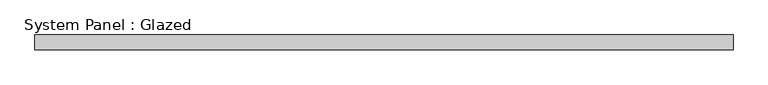
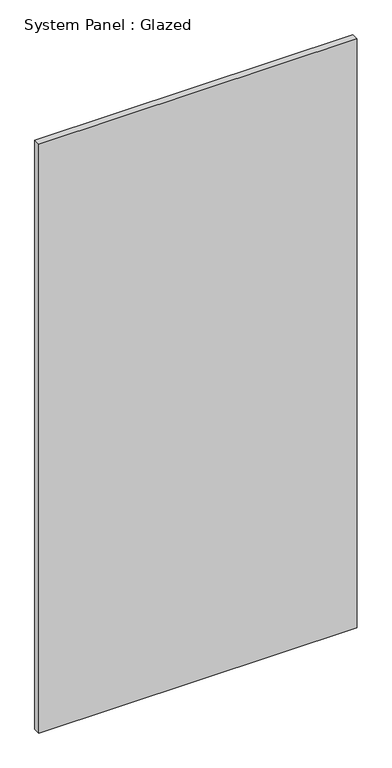
"""IFC4 building model written with IfcOpenShell, lengths in millimetres: plate geometry, System Panel : Glazed."""

import ifcopenshell
import ifcopenshell.guid

model = None  # the IFC model being written
_history = None  # IfcOwnerHistory: only IFC2X3 demands one
_inside = {}  # id of a spatial element -> (the spatial element, [elements in it])
_under = {}  # id of a project, library or spatial element -> (it, [spatial elements below it])
_declared = {}  # id of a project -> (the project, [libraries it declares])
_typed = {}  # id of a type object -> (the type object, [elements of that type])
_made_of = {}  # id of a material, layer set ... -> (it, [elements and type objects made of it])


def new_model(schema):
    """Start an empty IFC model of exactly this schema.

    Asked for "IFC4X3", IfcOpenShell would pick the latest addendum, in which some entities
    have other attributes; the version numbers below select the first issue.
    IFC2X3 requires an IfcOwnerHistory on every rooted entity: one is made here for all.
    """
    global model, _history
    if schema == "IFC4X3":
        model = ifcopenshell.file(schema_version=(4, 3, 0, 0))
    else:
        model = ifcopenshell.file(schema=schema)
    _inside.clear()
    _under.clear()
    _declared.clear()
    _typed.clear()
    _made_of.clear()
    _history = None
    if model.schema == "IFC2X3":
        org = make("IfcOrganization", Name="unknown")
        user = make(
            "IfcPersonAndOrganization",
            ThePerson=make("IfcPerson", FamilyName="unknown"),
            TheOrganization=org,
        )
        app = make(
            "IfcApplication",
            ApplicationDeveloper=org,
            Version="unknown",
            ApplicationFullName="unknown",
            ApplicationIdentifier="unknown",
        )
        _history = make(
            "IfcOwnerHistory",
            OwningUser=user,
            OwningApplication=app,
            ChangeAction="ADDED",
            CreationDate=0,
        )
    return model


def make(cls, **values):
    """One entity of the class cls with the attributes given. An attribute that is None is left unset."""
    return model.create_entity(
        cls, **{name: value for name, value in values.items() if value is not None}
    )


def rooted(cls, **values):
    """An entity with a GlobalId (a new one), such as an element, a storey or a relation."""
    return make(cls, GlobalId=ifcopenshell.guid.new(), OwnerHistory=_history, **values)


def si_unit(unit_type, name, prefix=None):
    """IfcSIUnit, for example si_unit("LENGTHUNIT", "METRE", prefix="MILLI")."""
    return make("IfcSIUnit", UnitType=unit_type, Prefix=prefix, Name=name)


def assignment(units):
    """IfcUnitAssignment: the units of a project."""
    return None if units is None else make("IfcUnitAssignment", Units=units)


def point(xyz):
    """IfcCartesianPoint."""
    return None if xyz is None else make("IfcCartesianPoint", Coordinates=xyz)


def direction(xyz):
    """IfcDirection."""
    return None if xyz is None else make("IfcDirection", DirectionRatios=xyz)


def frame(location, z_axis=None, x_axis=None):
    """IfcAxis2Placement3D, a coordinate frame: its origin and axes. An axis left out is left unset."""
    return make(
        "IfcAxis2Placement3D",
        Location=point(location),
        Axis=direction(z_axis),
        RefDirection=direction(x_axis),
    )


def origin():
    """The frame at (0, 0, 0) with its axes left unset."""
    return frame((0.0, 0.0, 0.0))


def origin_with_axes():
    """The frame at (0, 0, 0) with the z axis (0, 0, 1) and the x axis (1, 0, 0) written out."""
    return frame((0.0, 0.0, 0.0), z_axis=(0.0, 0.0, 1.0), x_axis=(1.0, 0.0, 0.0))


def place(relative_to, where):
    """IfcLocalPlacement: puts the frame where relative to a parent placement (None: the world)."""
    return make(
        "IfcLocalPlacement", PlacementRelTo=relative_to, RelativePlacement=where
    )


def context(
    kind, dimensions, precision=None, world=None, true_north=None, identifier=None
):
    """IfcGeometricRepresentationContext, for example the 3D "Model" context."""
    return make(
        "IfcGeometricRepresentationContext",
        ContextIdentifier=identifier,
        ContextType=kind,
        CoordinateSpaceDimension=dimensions,
        Precision=precision,
        WorldCoordinateSystem=world,
        TrueNorth=true_north,
    )


def project(units=None, contexts=None):
    """IfcProject with its units and contexts."""
    return rooted(
        "IfcProject",
        Name="project",
        RepresentationContexts=contexts,
        UnitsInContext=assignment(units),
    )


def spatial(cls, under=None, at=None, **own):
    """A site, building, storey or space (cls), placed at a placement, below another one or the project."""
    s = rooted(cls, ObjectPlacement=at, **own)
    if under is not None:
        _under.setdefault(under.id(), (under, []))[1].append(s)
    return s


def polyline(points):
    """IfcPolyline through the points."""
    return make("IfcPolyline", Points=[point(p) for p in points])


def outline(outer, holes=None, kind="AREA"):
    """IfcArbitraryClosedProfileDef: a profile drawn as a closed curve; with holes, ...WithVoids."""
    if holes is None:
        return make("IfcArbitraryClosedProfileDef", ProfileType=kind, OuterCurve=outer)
    return make(
        "IfcArbitraryProfileDefWithVoids",
        ProfileType=kind,
        OuterCurve=outer,
        InnerCurves=holes,
    )


def extrude(swept, where, along, depth):
    """IfcExtrudedAreaSolid: the profile swept, set in the frame where, extruded along a direction by depth."""
    return make(
        "IfcExtrudedAreaSolid",
        SweptArea=swept,
        Position=where,
        ExtrudedDirection=direction(along),
        Depth=depth,
    )


def shape(context_of_items, identifier, shape_type, items):
    """IfcShapeRepresentation: the items that make up one representation, for example the "Body"."""
    return make(
        "IfcShapeRepresentation",
        ContextOfItems=context_of_items,
        RepresentationIdentifier=identifier,
        RepresentationType=shape_type,
        Items=items,
    )


def source(mapping_origin, context_of_items, identifier, shape_type, items):
    """IfcRepresentationMap: a shape defined once, which mapped items show again and again."""
    return make(
        "IfcRepresentationMap",
        MappingOrigin=mapping_origin,
        MappedRepresentation=shape(context_of_items, identifier, shape_type, items),
    )


def transform(
    local_origin,
    x_axis=None,
    y_axis=None,
    z_axis=None,
    scale=None,
    scale2=None,
    scale3=None,
    uniform=True,
):
    """IfcCartesianTransformationOperator3D, or its non-uniform kind. x_axis, y_axis, z_axis: its Axis1, 2, 3."""
    if uniform:
        return make(
            "IfcCartesianTransformationOperator3D",
            Axis1=direction(x_axis),
            Axis2=direction(y_axis),
            LocalOrigin=point(local_origin),
            Scale=scale,
            Axis3=direction(z_axis),
        )
    return make(
        "IfcCartesianTransformationOperator3DnonUniform",
        Axis1=direction(x_axis),
        Axis2=direction(y_axis),
        LocalOrigin=point(local_origin),
        Scale=scale,
        Axis3=direction(z_axis),
        Scale2=scale2,
        Scale3=scale3,
    )


def mapped(mapping_source, mapping_target):
    """IfcMappedItem: shows the shape of a source again, moved by a transform."""
    return make(
        "IfcMappedItem", MappingSource=mapping_source, MappingTarget=mapping_target
    )


def made_of(thing, what):
    """Note that an element or type object is made of a material, layer set ...; save() writes the relation."""
    if what is not None:
        _made_of.setdefault(what.id(), (what, []))[1].append(thing)
    return thing


def element(
    cls,
    number,
    at=None,
    inside=None,
    cuts=None,
    type_object=None,
    material=None,
    context=None,
    identifier="Body",
    shape_type=None,
    held_by="IfcProductDefinitionShape",
    body=None,
    shapes=None,
    **own,
):
    """One element of the class cls, such as IfcWall. Its Tag is "e" and its number.

    at: its placement. inside: the storey or other place that contains it. cuts: it is an
    opening in that element (IfcRelVoidsElement). A single representation is given by context,
    identifier, shape_type and body (its items); several are given by shapes. held_by: the class
    of the entity that holds the representations. save() writes the other relations.
    """
    e = rooted(cls, Tag="e%d" % number, ObjectPlacement=at, **own)
    if body is not None:
        shapes = [shape(context, identifier, shape_type, body)]
    if shapes is not None:
        e.Representation = make(held_by, Representations=shapes)
    if inside is not None:
        _inside.setdefault(inside.id(), (inside, []))[1].append(e)
    if cuts is not None:
        rooted(
            "IfcRelVoidsElement", RelatingBuildingElement=cuts, RelatedOpeningElement=e
        )
    if type_object is not None:
        _typed.setdefault(type_object.id(), (type_object, []))[1].append(e)
    return made_of(e, material)


def aggregate(whole, parts):
    """IfcRelAggregates: a whole, such as a stair, and the parts it consists of."""
    return rooted("IfcRelAggregates", RelatingObject=whole, RelatedObjects=parts)


def save(model, path):
    """Write the relations noted so far, then the file.

    IfcRelAggregates (storeys below a building ...), IfcRelContainedInSpatialStructure (elements
    in a storey), IfcRelDefinesByType, IfcRelAssociatesMaterial and IfcRelDeclares: one each for
    every whole, place, type object, material and project.
    """
    for whole, parts in _under.values():
        aggregate(whole, parts)
    for where, things in _inside.values():
        rooted(
            "IfcRelContainedInSpatialStructure",
            RelatedElements=things,
            RelatingStructure=where,
        )
    for kind, things in _typed.values():
        rooted("IfcRelDefinesByType", RelatedObjects=things, RelatingType=kind)
    for what, things in _made_of.values():
        rooted("IfcRelAssociatesMaterial", RelatedObjects=things, RelatingMaterial=what)
    for by, libraries in _declared.values():
        rooted("IfcRelDeclares", RelatingContext=by, RelatedDefinitions=libraries)
    model.write(path)


def system_panel_glazed_cc393cf4(model_context):
    return source(origin(), model_context, "Body", "SweptSolid", [
        extrude(outline(polyline([(599.0166667, 19.05), (-599.0166667, 19.05), (-599.0166667, 44.45), (599.0166667, 44.45), (599.0166667, 19.05)])), origin_with_axes(), (0.0, 0.0, 1.0), 2343.15),
    ])


if __name__ == "__main__":
    model = new_model("IFC4")
    model_context = context("Model", 3, world=origin())
    ifc_project = project(units=[si_unit("LENGTHUNIT", "METRE", prefix="MILLI")], contexts=[model_context])
    site = spatial("IfcSite", under=ifc_project)
    building = spatial("IfcBuilding", under=site)
    placement = place(None, origin())
    system_panel_glazed_shape = system_panel_glazed_cc393cf4(model_context)
    element("IfcPlate", 1, ObjectType="System Panel : Glazed", at=placement, inside=building, context=model_context, shape_type="MappedRepresentation", body=[
        mapped(system_panel_glazed_shape, transform((0.0, 0.0, 0.0), x_axis=(1.0, 0.0, 0.0), y_axis=(0.0, 1.0, 0.0), z_axis=(0.0, 0.0, 1.0))),
    ])
    save(model, "model.ifc")

# Revit data of these elements
# Element 1 (IfcPlate, "System Panel : Glazed")
#   Materials on its faces: "Glass"
# Materials
#   "Glass": class "Glass", colour RGB 218 227 224, transparency 0.85, Description = "Soda Lime Glass", Cost = 0
